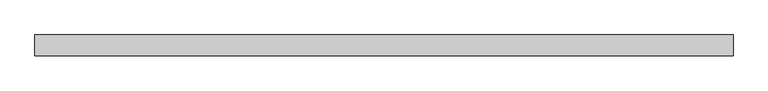
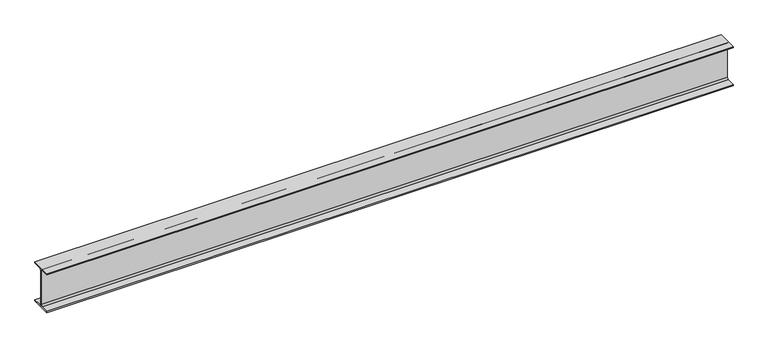
"""IFC4 building model written with IfcOpenShell, lengths in millimetres: beam geometry, 0912_Steel Framing_H-KSD3502 : H_SB_ASB_H-350x175x7x11."""

from ifc_helpers import new_model, si_unit, point, frame, frame_2d, origin, place, context, project, spatial, polyline, circle_curve, trimmed, segment, composite_curve, outline, extrude, source, transform, mapped, element, save


def beam_3979fe98(model_context):
    return source(origin(), model_context, "Body", "SweptSolid", [
        extrude(outline(composite_curve([segment(polyline([(87.5, -164.0), (87.5, -175.0), (-87.5, -175.0), (-87.5, -164.0), (-17.5, -164.0)]), True, "CONTINUOUS"), segment(trimmed(circle_curve(frame_2d((-17.5, -150.0)), 14.0), [point((-17.5, -164.0))], [point((-3.5, -150.0))], True, "CARTESIAN"), True, "CONTINUOUS"), segment(polyline([(-3.5, -150.0), (-3.5, 150.0)]), True, "CONTINUOUS"), segment(trimmed(circle_curve(frame_2d((-17.5, 150.0)), 14.0), [point((-3.5, 150.0))], [point((-17.5, 164.0))], True, "CARTESIAN"), True, "CONTINUOUS"), segment(polyline([(-17.5, 164.0), (-87.5, 164.0), (-87.5, 175.0), (87.5, 175.0), (87.5, 164.0), (17.5, 164.0)]), True, "CONTINUOUS"), segment(trimmed(circle_curve(frame_2d((17.5, 150.0)), 14.0), [point((17.5, 164.0))], [point((3.5, 150.0))], True, "CARTESIAN"), True, "CONTINUOUS"), segment(polyline([(3.5, 150.0), (3.5, -150.0)]), True, "CONTINUOUS"), segment(trimmed(circle_curve(frame_2d((17.5, -150.0)), 14.0), [point((3.5, -150.0))], [point((17.5, -164.0))], True, "CARTESIAN"), True, "CONTINUOUS"), segment(polyline([(17.5, -164.0), (87.5, -164.0)]), True, "CONTINUOUS")], self_intersect=False)), frame((-2889.9826898, 0.0, 0.0), z_axis=(1.0, 0.0, 0.0), x_axis=(0.0, 1.0, 0.0)), (0.0, 0.0, 1.0), 5810.1548079),
    ])


if __name__ == "__main__":
    model = new_model("IFC4")
    model_context = context("Model", 3, world=origin())
    ifc_project = project(units=[si_unit("LENGTHUNIT", "METRE", prefix="MILLI")], contexts=[model_context])
    site = spatial("IfcSite", under=ifc_project)
    building = spatial("IfcBuilding", under=site)
    placement = place(None, origin())
    beam_shape = beam_3979fe98(model_context)
    element("IfcBeam", 1, ObjectType="0912_Steel Framing_H-KSD3502 : H_SB_ASB_H-350x175x7x11", at=placement, inside=building, context=model_context, shape_type="MappedRepresentation", body=[
        mapped(beam_shape, transform((0.0, 0.0, 0.0), x_axis=(1.0, 0.0, 0.0), y_axis=(0.0, 1.0, 0.0), z_axis=(0.0, 0.0, 1.0))),
    ])
    save(model, "model.ifc")

# Revit data of these elements
# Type "0912_Steel Framing_H-KSD3502 : H_SB_ASB_H-350x175x7x11"
#   H_WM Code_1 = "S01AA002-00001 | Main Steel Structure Fabrication Work | Shelter/Building | Medium Steel - Standard (90KG/M>Weight≥30KG/M) | Material: (   )"
#   H_WM Code_2 = "S03AA028-00001 | Main Steel Structure Erection Work | Shelter/Building | Medium Steel (90KG/M>Weight≥30KG/M) | Material: (   )"
#   H_WM Code_3 = "S01AA010-00001 | Main Steel Structure Fabrication Work | Shelter/Building | Steel Painting/Coating | for Non-Fireproofed Steel Surface, Surface Preparation, Primer, Second & Final Coat | Material: (   )"
#   H_Q'ty Cal Type Tag = "SB-Q2"
#   Width = 17.5 cm
#   Web Thickness = 0.7 cm
#   Web Fillet = 1.4 cm
#   Warping Constant = 282000.0 cm⁶
#   W = 0
#   Torsional Moment of Inertia = 19.4042 cm⁴
#   Section Area = 63.14 cm²
#   Plastic Modulus weak axis = 174.0 cm³
#   Plastic Modulus strong axis = 868.0 cm³
#   Perimeter = 1.36 m²/m
#   Nominal Weight = 49.60 kgf/m
#   Moment of Inertia weak axis = 984.00 cm⁴
#   Moment of Inertia strong axis = 13600.00 cm⁴
#   Height = 35.0 cm
#   Flange Thickness = 1.1 cm
#   Elastic Modulus weak axis = 112.0 cm³
#   Elastic Modulus strong axis = 775.0 cm³
#   Centroid Vertical = 17.5 cm
#   Centroid Horizontal = 8.75 cm
#   Ix = 136000000
#   Length [instance default] = 1.5240 m
#   Zx = 868000
#   b = 0.1750 m
#   h = 0.3500 m
#   r = 0.0140 m
#   s = 0.0070 m
#   t = 0.0110 m
#   A = 0.006314 m²
#   Structural Material [instance default] = Steel, 45-345
#   Assembly Code = ""
# Element 1 (IfcBeam, "0912_Steel Framing_H-KSD3502 : H_SB_ASB_H-350x175x7x11")
#   Structural Material = none
# Materials
#   "Steel, 45-345": class "Metal", colour RGB 189 187 185, transparency 0, Description = "Steel 345 MPa", Cost = 0
